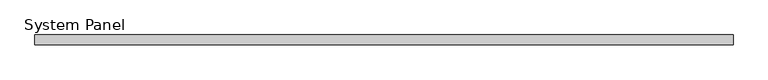
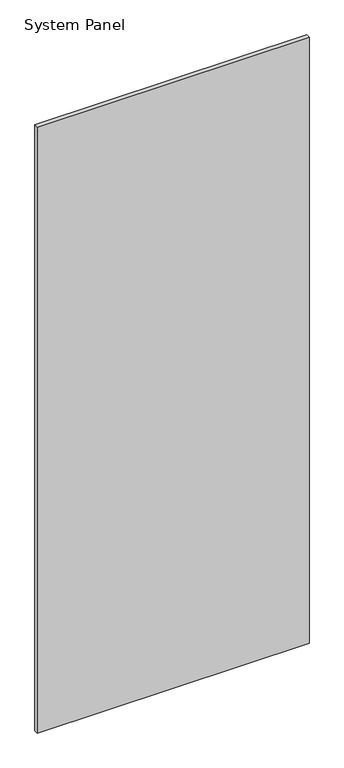
"""IFC4 building model written with IfcOpenShell, lengths in millimetres: plate geometry, System Panel : WWm-Glass-20mm-10mmOffset."""

from ifc_helpers import new_model, si_unit, origin, origin_with_axes, place, context, project, spatial, polyline, outline, extrude, source, transform, mapped, element, save


def system_panel_fa7b2e37(model_context):
    return source(origin(), model_context, "Body", "SweptSolid", [
        extrude(outline(polyline([(711.0919118, 0.0), (-711.0919118, 0.0), (-711.0919118, 20.0), (711.0919118, 20.0), (711.0919118, 0.0)])), origin_with_axes(), (0.0, 0.0, 1.0), 3350.0),
    ])


if __name__ == "__main__":
    model = new_model("IFC4")
    model_context = context("Model", 3, world=origin())
    ifc_project = project(units=[si_unit("LENGTHUNIT", "METRE", prefix="MILLI")], contexts=[model_context])
    site = spatial("IfcSite", under=ifc_project)
    building = spatial("IfcBuilding", under=site)
    placement = place(None, origin())
    system_panel_shape = system_panel_fa7b2e37(model_context)
    element("IfcPlate", 1, ObjectType="System Panel : WWm-Glass-20mm-10mmOffset", at=placement, inside=building, context=model_context, shape_type="MappedRepresentation", body=[
        mapped(system_panel_shape, transform((0.0, 0.0, 0.0), x_axis=(1.0, 0.0, 0.0), y_axis=(0.0, 1.0, 0.0), z_axis=(0.0, 0.0, 1.0))),
    ])
    save(model, "model.ifc")

# Revit data of these elements
# Type "System Panel : WWm-Glass-20mm-10mmOffset"
#   Finish = ""
# Element 1 (IfcPlate, "System Panel : WWm-Glass-20mm-10mmOffset")
#   Materials on its faces: "WW-EC-GL-Storefront"
# Materials
#   "WW-EC-GL-Storefront": class "Glass", colour RGB 236 240 239, transparency 0.85, Description = "Storefront Glass", Cost = 0
